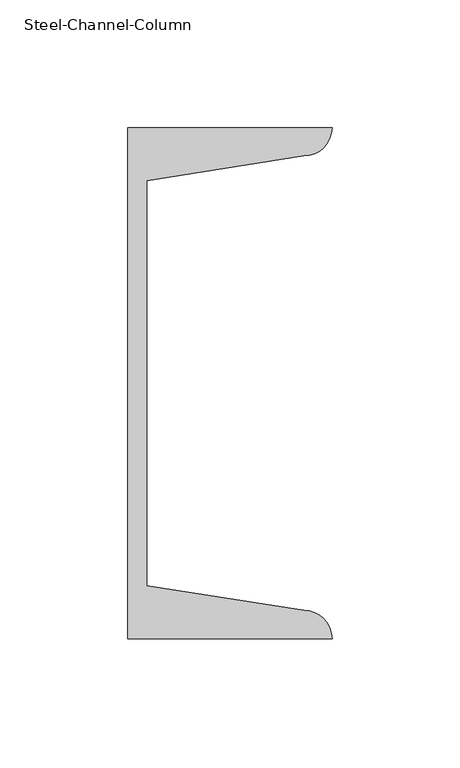
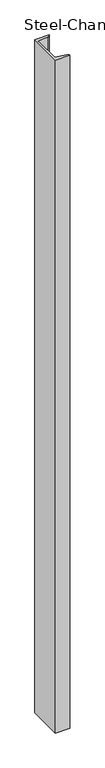
"""IFC4 building model written with IfcOpenShell, lengths in millimetres: column geometry, Steel-Channel-Column : CL126_C-200×80x7.5x11."""

from ifc_helpers import new_model, si_unit, point, frame_2d, origin, origin_with_axes, place, context, project, spatial, polyline, circle_curve, trimmed, segment, composite_curve, outline, extrude, source, transform, mapped, element, save


def steel_channel_column_12e21b6e(model_context):
    return source(origin(), model_context, "Body", "SweptSolid", [
        extrude(outline(composite_curve([segment(polyline([(-22.1, 100.0), (57.9, 100.0)]), True, "CONTINUOUS"), segment(trimmed(circle_curve(frame_2d((46.9, 100.0)), 11.0), [point((57.9, 100.0))], [point((46.9, 89.0))], False, "CARTESIAN"), True, "CONTINUOUS"), segment(polyline([(46.9, 89.0), (-14.6, 79.2593569), (-14.6, -79.2593569), (46.9, -89.0)]), True, "CONTINUOUS"), segment(trimmed(circle_curve(frame_2d((46.9, -100.0)), 11.0), [point((46.9, -89.0))], [point((57.9, -100.0))], False, "CARTESIAN"), True, "CONTINUOUS"), segment(polyline([(57.9, -100.0), (-22.1, -100.0), (-22.1, 100.0)]), True, "CONTINUOUS")], self_intersect=False)), origin_with_axes(), (0.0, 0.0, 1.0), 4000.0),
    ])


if __name__ == "__main__":
    model = new_model("IFC4")
    model_context = context("Model", 3, world=origin())
    ifc_project = project(units=[si_unit("LENGTHUNIT", "METRE", prefix="MILLI")], contexts=[model_context])
    site = spatial("IfcSite", under=ifc_project)
    building = spatial("IfcBuilding", under=site)
    placement = place(None, origin())
    steel_channel_column_shape = steel_channel_column_12e21b6e(model_context)
    element("IfcColumn", 1, ObjectType="Steel-Channel-Column : CL126_C-200×80x7.5x11", at=placement, inside=building, context=model_context, shape_type="MappedRepresentation", body=[
        mapped(steel_channel_column_shape, transform((0.0, 0.0, 0.0), x_axis=(1.0, 0.0, 0.0), y_axis=(0.0, 1.0, 0.0), z_axis=(0.0, 0.0, 1.0))),
    ])
    save(model, "model.ifc")

# Revit data of these elements
# Project information
#   Project ISM Data = "<?xml version=\"1.0\" encoding=\"utf-16\"?><ism schema_version=\"03.00\"><section_positioning><element family_name=\"CO_RC_REC\" symbol_name=\"CCC12_Rec_450x450\" section_id=\"F2ADF140-E21A-4820-8170-6F63D956DCAD\" category=\"OST_StructuralColumns\" mirror_y=\"0\" mirror_x=\"0\" /><element family_name=\"CO_RC_REC\" symbol_name=\"CCC12_Rec_450x450\" section_id=\"B35A310E-4F33-462b-819C-3ADD300C0CEB\" category=\"OST_StructuralColumns\" mirror_y=\"0\" mirror_x=\"0\" /><element family_name=\"CO_RC_REC\" symbol_name=\"CCC12_Rec_450x450\" section_id=\"711054EC-0DB2-46e3-AD20-004560300C00\" category=\"OST_StructuralColumns\" mirror_y=\"0\" mirror_x=\"0\" /><element family_name=\"CO_RC_REC\" symbol_name=\"300 x 450\" section_id=\"B5C54EC9-8EBD-4860-AB72-EF5791AED394\" category=\"OST_StructuralColumns\" mirror_y=\"0\" mirror_x=\"0\" /><element family_name=\"GI_RC_C\" symbol_name=\"SGC11_400x500\" section_id=\"0A7B8D02-9EA4-4aa9-A41A-E30BB5B6B6C5\" category=\"OST_StructuralFraming\" mirror_y=\"0\" mirror_x=\"0\" /><element family_name=\"GI_RC_C\" symbol_name=\"SGC11_400x500\" section_id=\"714BBD27-DB58-47da-B54C-5806291C2D3C\" category=\"OST_StructuralFraming\" mirror_y=\"0\" mirror_x=\"0\" /><element family_name=\"GI_RC_C\" symbol_name=\"SGC11_400x500\" section_id=\"F36E62C1-13EE-4807-A3C1-899E23E0BEDE\" category=\"OST_StructuralFraming\" mirror_y=\"0\" mirror_x=\"0\" /><element family_name=\"GI_RC_C\" symbol_name=\"SGC11_400x500\" section_id=\"F5448801-679E-44d6-8F46-E676344F8165\" category=\"OST_StructuralFraming\" mirror_y=\"0\" mirror_x=\"0\" /><element family_name=\"GI_RC_C\" symbol_name=\"SGC11_400x600\" section_id=\"05D74241-6318-4cac-95F5-7B878260D5B5\" category=\"OST_StructuralFraming\" mirror_y=\"0\" mirror_x=\"0\" /><element family_name=\"GI_RC_C\" symbol_name=\"SGC11_400x500\" section_id=\"846DCB0C-E06B-4978-9D43-E1CC0FDE7595\" category=\"OST_StructuralFraming\" mirror_y=\"0\" mirror_x=\"0\" /><element family_name=\"GI_RC_C\" symbol_name=\"SGC11_400x500\" section_id=\"2ADF82B8-986D-4f44-85DE-89D921292160\" category=\"OST_StructuralFraming\" mirror_y=\"0\" mirror_x=\"0\" /><element family_name=\"GI_RC_C\" symbol_name=\"SGC11_400x500\" section_id=\"7AF371ED-051B-4a30-8826-11F11C212B73\" category=\"OST_StructuralFraming\" mirror_y=\"0\" mirror_x=\"0\" /><element family_name=\"GI_RC_C\" symbol_name=\"SGC11_400x500\" section_id=\"2FE74006-ADDA-412f-A522-853919E62B4D\" category=\"OST_StructuralFraming\" mirror_y=\"0\" mirror_x=\"0\" /><element family_name=\"GI_RC_C\" symbol_name=\"SGC11_400x500\" section_id=\"09B63641-D581-4a6c-A18E-54C17EC989A4\" category=\"OST_StructuralFraming\" mirror_y=\"0\" mirror_x=\"0\" /><element family_name=\"GI_RC_C\" symbol_name=\"SGC11_400x500\" section_id=\"0DD6B52A-77D0-45a1-82B1-8236ED57078C\" category=\"OST_StructuralFraming\" mirror_y=\"0\" mirror_x=\"0\" /><element family_name=\"GI_RC_C\" symbol_name=\"SGC11_400x500\" section_id=\"35D311D2-DEB8-4469-97DE-110B6DF5B84D\" category=\"OST_StructuralFraming\" mirror_y=\"0\" mirror_x=\"0\" /><element family_name=\"GI_RC_C\" symbol_name=\"SGC11_400x500\" section_id=\"0D3CCDE5-CFF9-431b-A4BD-01BF6636D6BD\" category=\"OST_StructuralFraming\" mirror_y=\"0\" mirror_x=\"0\" /><element family_name=\"GI_RC_C\" symbol_name=\"SGC11_400x500\" section_id=\"C62B2A5B-024A-47ac-B030-C17A67E64A7B\" category=\"OST_StructuralFraming\" mirror_y=\"0\" mirror_x=\"0\" /><element family_name=\"GI_RC_C\" symbol_name=\"SGC11_400x500\" section_id=\"944C6E43-E607-48c3-8358-9E6CB88346E7\" category=\"OST_StructuralFraming\" mirror_y=\"0\" mirror_x=\"0\" /><element family_name=\"GI_RC_C\" symbol_name=\"SGC11_400x500\" section_id=\"A4B1F42D-B1C2-4ad2-8AD6-DB0D5E05998D\" category=\"OST_StructuralFraming\" mirror_y=\"0\" mirror_x=\"0\" /><element family_name=\"GI_RC_C\" symbol_name=\"SGC11_400x500\" section_id=\"007E6C70-1139-4b48-B003-C76FAD4C249A\" category=\"OST_StructuralFraming\" mirror_y=\"0\" mirror_x=\"0\" /><element family_name=\"GI_RC_C\" symbol_name=\"SGC11_400x500\" section_id=\"9941AC94-F03A-464c-9912-04590E0C31E0\" category=\"OST_StructuralFraming\" mirror_y=\"0\" mirror_x=\"0\" /><element family_name=\"GI_RC_C\" symbol_name=\"SGC11_400x500\" section_id=\"CFD98B8D-8FF4-4e71-A909-0FE7DBCE924E\" category=\"OST_StructuralFraming\" mirror_y=\"0\" mirror_x=\"0\" /><element family_name=\"GI_RC_C\" symbol_name=\"SGC11_400x500\" section_id=\"58262161-98E6-45c8-B2BD-4508105FF662\" category=\"OST_StructuralFraming\" mirror_y=\"0\" mirror_x=\"0\" /><element family_name=\"GI_RC_C\" symbol_name=\"SGC11_400x500\" section_id=\"66AB4841-610A-4883-97F7-1282A56484E1\" category=\"OST_StructuralFraming\" mirror_y=\"0\" mirror_x=\"0\" /><element family_name=\"GI_RC_C\" symbol_name=\"SGC11_400x500\" section_id=\"D2B324BE-BBD6-49da-9730-60EA7AD4D3A0\" category=\"OST_StructuralFraming\" mirror_y=\"0\" mirror_x=\"0\" /><element family_name=\"GI_RC_C\" symbol_name=\"SGC11_400x500\" section_id=\"92A8ECE7-C053-46b1-92ED-F2C041617E7B\" category=\"OST_StructuralFraming\" mirror_y=\"0\" mirror_x=\"0\" /><element family_name=\"GI_RC_C\" symbol_name=\"SGC11_400x500\" section_id=\"B4C4BDB0-65C4-4016-9C78-DBD77E229523\" category=\"OST_StructuralFraming\" mirror_y=\"0\" mirror_x=\"0\" /><element family_name=\"GI_RC_C\" symbol_name=\"SGC11_400x500\" section_id=\"57270646-162F-4c83-BDB7-A5FBEA9120BD\" category=\"OST_StructuralFraming\" mirror_y=\"0\" mirror_x=\"0\" /><element family_name=\"GI_RC_C\" symbol_name=\"SGC11_400x500\" section_id=\"BDEF733F-00AA-4eee-B6C6-50229FC1D236\" category=\"OST_StructuralFraming\" mirror_y=\"0\" mirror_x=\"0\" /><element family_name=\"GI_RC_C\" symbol_name=\"SGC11_400x500\" section_id=\"84A94E1E-3074-40f4-9690-97191755F019\" category=\"OST_StructuralFraming\" mirror_y=\"0\" mirror_x=\"0\" /><element family_name=\"GI_RC_C\" symbol_name=\"SGC11_400x500\" section_id=\"8A7D913D-7967-4718-912D-B83DF0AD2EDD\" category=\"OST_StructuralFraming\" mirror_y=\"0\" mirror_x=\"0\" /><element family_name=\"GI_RC_C\" symbol_name=\"SGC11_400x500\" section_id=\"83553D70-90FA-469c-B5C3-EF03F3FC6475\" category=\"OST_StructuralFraming\" mirror_y=\"0\" mirror_x=\"0\" /><element family_name=\"GI_RC_C\" symbol_name=\"SGC11_400x500\" section_id=\"6880C1E4-C50B-4c1b-B61C-23F2D8C46873\" category=\"OST_StructuralFraming\" mirror_y=\"0\" mirror_x=\"0\" /><element family_name=\"GI_RC_C\" symbol_name=\"SGC11_400x500\" section_id=\"08594C43-CD40-47de-A3BA-8BFB47F64994\" category=\"OST_StructuralFraming\" mirror_y=\"0\" mirror_x=\"0\" /><element family_name=\"GI_RC_C\" symbol_name=\"SGC11_400x500\" section_id=\"7D2E11FA-A5E1-4434-B9BE-AABA1A16CA03\" category=\"OST_StructuralFraming\" mirror_y=\"0\" mirror_x=\"0\" /><element family_name=\"GI_RC_C\" symbol_name=\"SGC11_400x500\" section_id=\"D892DFA4-5441-4ad2-A390-253492293B1B\" category=\"OST_StructuralFraming\" mirror_y=\"0\" mirror_x=\"0\" /><element family_name=\"GI_RC_C\" symbol_name=\"SGC11_400x500\" section_id=\"E5A32FE6-89C4-49f1-B3B9-1CABE7C48A4D\" category=\"OST_StructuralFraming\" mirror_y=\"0\" mirror_x=\"0\" /><element family_name=\"GI_RC_C\" symbol_name=\"SGC11_400x500\" section_id=\"8AE872C2-5DBE-47c5-934B-7E964A84B589\" category=\"OST_StructuralFraming\" mirror_y=\"0\" mirror_x=\"0\" /><element family_name=\"GI_RC_C\" symbol_name=\"SGC11_400x500\" section_id=\"3C847B60-488A-4604-A400-16A3A65E919B\" category=\"OST_StructuralFraming\" mirror_y=\"0\" mirror_x=\"0\" /><element family_name=\"GI_RC_C\" symbol_name=\"SGC11_400x500\" section_id=\"DBEC432A-3F7B-4266-AD99-2A937DC70BCF\" category=\"OST_StructuralFraming\" mirror_y=\"0\" mirror_x=\"0\" /><element family_name=\"GI_RC_C\" symbol_name=\"SGC11_400x500\" section_id=\"59403DD6-7A51-48aa-A3BE-962457E6F10E\" category=\"OST_StructuralFraming\" mirror_y=\"0\" mirror_x=\"0\" /><element family_name=\"GI_RC_C\" symbol_name=\"SGC11_400x500\" section_id=\"11CDDF5D-38B6-43b2-A291-FC188BE232BC\" category=\"OST_StructuralFraming\" mirror_y=\"0\" mirror_x=\"0\" /><element family_name=\"GI_RC_C\" symbol_name=\"SGC11_400x500\" section_id=\"10BF2843-EFC9-4136-933C-5B270D970277\" category=\"OST_StructuralFraming\" mirror_y=\"0\" mirror_x=\"0\" /><element family_name=\"GI_RC_C\" symbol_name=\"SGC11_400x500\" section_id=\"E1B09A9C-F6C6-47d9-976B-E313C0E3F52B\" category=\"OST_StructuralFraming\" mirror_y=\"0\" mirror_x=\"0\" /><element family_name=\"GI_RC_C\" symbol_name=\"SGC11_400x500\" section_id=\"A3A22EC3-26C8-4588-A0AB-AFAE02DF267E\" category=\"OST_StructuralFraming\" mirror_y=\"0\" mirror_x=\"0\" /><element family_name=\"GI_RC_C\" symbol_name=\"SGC11_400x500\" section_id=\"114828FC-BDC1-4343-9119-BCB5395DAA64\" category=\"OST_StructuralFraming\" mirror_y=\"0\" mirror_x=\"0\" /><element family_name=\"GI_RC_C\" symbol_name=\"SGC11_400x500\" section_id=\"797626F9-3558-4623-826F-15FB93088CB3\" category=\"OST_StructuralFraming\" mirror_y=\"0\" mirror_x=\"0\" /><element family_name=\"GI_RC_C\" symbol_name=\"SGC11_400x500\" section_id=\"4BF369CD-DF09-4346-96CB-C6C6380A2599\" category=\"OST_StructuralFraming\" mirror_y=\"0\" mirror_x=\"0\" /><element family_name=\"GI_RC_C\" symbol_name=\"SGC11_400x500\" section_id=\"722B46BA-61C4-44a1-9ECF-325B60B6688D\" category=\"OST_StructuralFraming\" mirror_y=\"0\" mirror_x=\"0\" /><element family_name=\"GI_RC_C\" symbol_name=\"SGC11_400x500\" section_id=\"C33DBE84-19C1-4379-AB6E-A41F7420F18C\" category=\"OST_StructuralFraming\" mirror_y=\"0\" mirror_x=\"0\" /><element family_name=\"GI_RC_C\" symbol_name=\"SGC11_400x500\" section_id=\"1F2D3B75-66F2-4d88-A1DD-647969477B86\" category=\"OST_StructuralFraming\" mirror_y=\"0\" mirror_x=\"0\" /><element family_name=\"GI_RC_C\" symbol_name=\"SGC11_400x500\" section_id=\"DFBF96B2-410A-4f39-80C4-D8CF78561C93\" category=\"OST_StructuralFraming\" mirror_y=\"0\" mirror_x=\"0\" /><element family_name=\"GI_RC_C\" symbol_name=\"SGC11_400x500\" section_id=\"D6793CD3-AB64-417c-9C28-8B18A0A2D336\" category=\"OST_StructuralFraming\" mirror_y=\"0\" mirror_x=\"0\" /><element family_name=\"GI_RC_C\" symbol_name=\"SGC11_400x500\" section_id=\"90884AC0-EA00-4caa-86E1-E6B886FD90ED\" category=\"OST_StructuralFraming\" mirror_y=\"0\" mirror_x=\"0\" /><element family_name=\"GI_RC_C\" symbol_name=\"SGC11_400x500\" section_id=\"64BC7B89-F7C8-4dae-A5C8-F10DF9E5F6BA\" category=\"OST_StructuralFraming\" mirror_y=\"0\" mirror_x=\"0\" /><element family_name=\"GI_RC_C\" symbol_name=\"SGC11_400x500\" section_id=\"D82E4D85-2728-40e5-9F60-1C7FB2990D78\" category=\"OST_StructuralFraming\" mirror_y=\"0\" mirror_x=\"0\" /><element family_name=\"GI_RC_C\" symbol_name=\"SGC11_400x500\" section_id=\"1E6D05B9-BF84-4669-AA27-948ADA1D511E\" category=\"OST_StructuralFraming\" mirror_y=\"0\" mirror_x=\"0\" /><element family_name=\"GI_RC_C\" symbol_name=\"SGC11_400x500\" section_id=\"73608CB2-EB94-466e-883D-814030EF49D6\" category=\"OST_StructuralFraming\" mirror_y=\"0\" mirror_x=\"0\" /><element family_name=\"GI_RC_C\" symbol_name=\"SGC11_400x500\" section_id=\"4EAF07EF-4E08-4065-9F08-BF69D4413867\" category=\"OST_StructuralFraming\" mirror_y=\"1\" mirror_x=\"1\" /></section_positioning><surface_member_mappings /><element_binding><element revit_id=\"0aa8b22b-49cd-4eb2-b994-d423f7aad482-0014435e\" ism_id=\"637A3C89-B4B9-4EE4-9E04-FF73E7A5771D\" /><element revit_id=\"af7cfdda-f71a-4a09-bb03-63e0c16d5d93-00152efa\" ism_id=\"088C1743-AFAE-4D55-B14F-2330F3A79060\" /><element revit_id=\"af7cfdda-f71a-4a09-bb03-63e0c16d5d93-00152efc\" ism_id=\"38278b30-864a-4bde-bfee-6c2d4309b281\" /><element revit_id=\"af7cfdda-f71a-4a09-bb03-63e0c16d5d93-00152eff\" ism_id=\"e2895b00-887b-4cf1-92a9-c4855f67b579\" /><element revit_id=\"af7cfdda-f71a-4a09-bb03-63e0c16d5d93-00152f02\" ism_id=\"a6b13b86-1938-47ee-8937-754844bb71d9\" /><element revit_id=\"af7cfdda-f71a-4a09-bb03-63e0c16d5d93-00152f05\" ism_id=\"b3cdb4ae-01be-49a8-8521-dfb37fcb7a09\" /><element revit_id=\"af7cfdda-f71a-4a09-bb03-63e0c16d5d93-00152f08\" ism_id=\"0a200294-2d0f-43b2-a10b-c345be42008c\" /><element revit_id=\"af7cfdda-f71a-4a09-bb03-63e0c16d5d
#     93-00152f0a\" ism_id=\"434ac00d-0b75-408a-b526-bf8655b26baf\" /><element revit_id=\"af7cfdda-f71a-4a09-bb03-63e0c16d5d93-00152f0c\" ism_id=\"5e4f7e2a-2154-47cc-93bc-24e7bd197632\" /><element revit_id=\"af7cfdda-f71a-4a09-bb03-63e0c16d5d93-00152f0e\" ism_id=\"f1998cd9-044c-4f7a-99e6-248bc5b45dba\" /><element revit_id=\"af7cfdda-f71a-4a09-bb03-63e0c16d5d93-00152f10\" ism_id=\"6ca0e144-6dd7-4824-b6a4-c3599ffcc64c\" /><element revit_id=\"af7cfdda-f71a-4a09-bb03-63e0c16d5d93-00152f12\" ism_id=\"173f1f07-ca52-4750-b7f6-1ef0180c36ba\" /><element revit_id=\"af7cfdda-f71a-4a09-bb03-63e0c16d5d93-00152f15\" ism_id=\"29a619d1-86ac-46c7-a220-2e78769b313e\" /><element revit_id=\"af7cfdda-f71a-4a09-bb03-63e0c16d5d93-00152f17\" ism_id=\"de21b25d-6b5e-4da6-89ee-8b671f1287ec\" /><element revit_id=\"af7cfdda-f71a-4a09-bb03-63e0c16d5d93-00152f19\" ism_id=\"70cdf538-eeaa-48c4-9315-181e56578638\" /><element revit_id=\"af7cfdda-f71a-4a09-bb03-63e0c16d5d93-00152f1b\" ism_id=\"49734cf8-a963-4163-b104-a25bff74fff0\" /><element revit_id=\"af7cfdda-f71a-4a09-bb03-63e0c16d5d93-00152f1d\" ism_id=\"a5a98e28-e98d-4759-bcab-d40632bfc19f\" /><element revit_id=\"af7cfdda-f71a-4a09-bb03-63e0c16d5d93-00152f1f\" ism_id=\"ab6af08f-90da-4d2f-a66a-db65621b8e94\" /><element revit_id=\"af7cfdda-f71a-4a09-bb03-63e0c16d5d93-00152f21\" ism_id=\"a65b64ab-134d-4223-82b7-5e66d90bc276\" /><element revit_id=\"af7cfdda-f71a-4a09-bb03-63e0c16d5d93-00152f23\" ism_id=\"6a1f317f-8940-4af8-9522-8e6c47c0c3a6\" /><element revit_id=\"af7cfdda-f71a-4a09-bb03-63e0c16d5d93-00152f25\" ism_id=\"880c6aab-7058-4382-9d83-6c759bdcf822\" /><element revit_id=\"af7cfdda-f71a-4a09-bb03-63e0c16d5d93-00152f27\" ism_id=\"555977b1-6494-4ee8-b235-8bae97762787\" /><element revit_id=\"af7cfdda-f71a-4a09-bb03-63e0c16d5d93-00152f29\" ism_id=\"66c9b467-8c65-4f1e-9542-95b43d793e9b\" /><element revit_id=\"af7cfdda-f71a-4a09-bb03-63e0c16d5d93-00152f2b\" ism_id=\"217a9ce2-64ab-4115-836e-06014fa1b21e\" /><element revit_id=\"af7cfdda-f71a-4a09-bb03-63e0c16d5d93-00152f2d\" ism_id=\"f7fc30da-832d-44e7-bab3-dd115d25639e\" /><element revit_id=\"af7cfdda-f71a-4a09-bb03-63e0c16d5d93-00152f2f\" ism_id=\"715eb46c-1b8d-4226-a7c6-6c6c165bf34d\" /><element revit_id=\"af7cfdda-f71a-4a09-bb03-63e0c16d5d93-00152f31\" ism_id=\"ef53c2b2-6fcf-42d2-96ea-f30a899bf64f\" /><element revit_id=\"af7cfdda-f71a-4a09-bb03-63e0c16d5d93-00152f34\" ism_id=\"1aefa093-18ee-4a97-8178-1b1fb4b7aceb\" /><element revit_id=\"af7cfdda-f71a-4a09-bb03-63e0c16d5d93-00152f38\" ism_id=\"262f02a9-64ca-487b-befd-4b58d44dffa7\" /><element revit_id=\"af7cfdda-f71a-4a09-bb03-63e0c16d5d93-00152f3b\" ism_id=\"6f2442a8-c4c0-4b53-9d7f-7059d6ededd2\" /><element revit_id=\"af7cfdda-f71a-4a09-bb03-63e0c16d5d93-00152f3e\" ism_id=\"dd838df4-69c7-406c-93e1-418c01f5734f\" /><element revit_id=\"af7cfdda-f71a-4a09-bb03-63e0c16d5d93-00152f40\" ism_id=\"9dec5077-28a7-4c32-95d2-08813de6a916\" /><element revit_id=\"af7cfdda-f71a-4a09-bb03-63e0c16d5d93-00152f42\" ism_id=\"9370ae5f-9277-4bb3-917b-cb3f318800a8\" /><element revit_id=\"af7cfdda-f71a-4a09-bb03-63e0c16d5d93-00152f44\" ism_id=\"0f3f2c81-58b4-4698-b1be-75061a4a2ae1\" /><element revit_id=\"af7cfdda-f71a-4a09-bb03-63e0c16d5d93-00152f46\" ism_id=\"95dca10f-6510-4ae7-a23e-7a1fd6939662\" /><element revit_id=\"af7cfdda-f71a-4a09-bb03-63e0c16d5d93-00152f49\" ism_id=\"83bad907-6a1c-4702-9990-a1a9c13d0160\" /><element revit_id=\"af7cfdda-f71a-4a09-bb03-63e0c16d5d93-00152f4d\" ism_id=\"7dba72dc-0de8-457c-8d3c-9c80941133ff\" /><element revit_id=\"af7cfdda-f71a-4a09-bb03-63e0c16d5d93-00152f51\" ism_id=\"a6cf3de2-949b-45b4-8029-061e06e5ab91\" /><element revit_id=\"af7cfdda-f71a-4a09-bb03-63e0c16d5d93-00152f54\" ism_id=\"77af5754-dd62-4c90-accb-d0b9405b5baf\" /><element revit_id=\"af7cfdda-f71a-4a09-bb03-63e0c16d5d93-00152f56\" ism_id=\"6461cb37-823d-49bb-bea2-3dbd4db85a81\" /><element revit_id=\"af7cfdda-f71a-4a09-bb03-63e0c16d5d93-00152f59\" ism_id=\"e2f2909f-27bc-426e-b2db-27b1217d3560\" /><element revit_id=\"af7cfdda-f71a-4a09-bb03-63e0c16d5d93-00152f5b\" ism_id=\"46c410de-fc65-4593-ae24-da1a154b45fb\" /><element revit_id=\"af7cfdda-f71a-4a09-bb03-63e0c16d5d93-00152f5d\" ism_id=\"d7d73cf7-a31f-421c-bc39-3ba338a334b1\" /><element revit_id=\"af7cfdda-f71a-4a09-bb03-63e0c16d5d93-00152f61\" ism_id=\"6bd81f7b-5fd8-4f19-ad3a-4e009274854c\" /><element revit_id=\"af7cfdda-f71a-4a09-bb03-63e0c16d5d93-00152f64\" ism_id=\"f25b9af0-504f-4aaf-a359-d2bc9d32b683\" /><element revit_id=\"af7cfdda-f71a-4a09-bb03-63e0c16d5d93-00152f66\" ism_id=\"f143dcd3-1cc7-47ae-b4ed-c960a7d1349c\" /><element revit_id=\"af7cfdda-f71a-4a09-bb03-63e0c16d5d93-00152f68\" ism_id=\"296e8d7f-a89b-405a-b793-fc1ea4b11be5\" /><element revit_id=\"af7cfdda-f71a-4a09-bb03-63e0c16d5d93-00152f6b\" ism_id=\"48b24488-3184-439c-b285-73e81edfef17\" /><element revit_id=\"af7cfdda-f71a-4a09-bb03-63e0c16d5d93-00152f6e\" ism_id=\"0db0ccd4-631c-4972-aad8-2fd483c55629\" /><element revit_id=\"af7cfdda-f71a-4a09-bb03-63e0c16d5d93-00152f71\" ism_id=\"ee51bd40-01d8-4a48-92c6-90509a96cad2\" /><element revit_id=\"af7cfdda-f71a-4a09-bb03-63e0c16d5d93-00152f73\" ism_id=\"e5c66ce6-ca9d-4591-9d75-5348307a88bc\" /><element revit_id=\"af7cfdda-f71a-4a09-bb03-63e0c16d5d93-00152f75\" ism_id=\"892d82ae-6f73-4af5-8575-78955f2b6c3b\" /><element revit_id=\"af7cfdda-f71a-4a09-bb03-63e0c16d5d93-00152f78\" ism_id=\"cb5b2a2e-5551-4b87-9d0b-6382c09e6ce2\" /><element revit_id=\"af7cfdda-f71a-4a09-bb03-63e0c16d5d93-00152f7c\" ism_id=\"1177c4ab-d04b-426b-80ba-afa1f1403e20\" /><element revit_id=\"af7cfdda-f71a-4a09-bb03-63e0c16d5d93-00152f7f\" ism_id=\"235d8a18-f10a-44ad-8945-ebb2f02646fa\" /><element revit_id=\"af7cfdda-f71a-4a09-bb03-63e0c16d5d93-00152f83\" ism_id=\"6127db9d-7d4b-44c8-806c-e4f7d278db0c\" /><element revit_id=\"af7cfdda-f71a-4a09-bb03-63e0c16d5d93-00152f86\" ism_id=\"85d79da8-d317-4e5b-88a2-88d20cb73d7d\" /><element revit_id=\"af7cfdda-f71a-4a09-bb03-63e0c16d5d93-00152f89\" ism_id=\"f4105a19-7c5e-4970-9446-50e578b67af2\" /><element revit_id=\"af7cfdda-f71a-4a09-bb03-63e0c16d5d93-00152f8b\" ism_id=\"ab299061-87b1-4edc-8a5c-c55542368f39\" /><element revit_id=\"af7cfdda-f71a-4a09-bb03-63e0c16d5d93-00152f8d\" ism_id=\"43097401-25be-48d4-a7ba-f3c37c1b84e9\" /><element revit_id=\"af7cfdda-f71a-4a09-bb03-63e0c16d5d93-00152f8f\" ism_id=\"fd9214b7-59e9-4736-b544-a37d4c180e24\" /><element revit_id=\"af7cfdda-f71a-4a09-bb03-63e0c16d5d93-00152f91\" ism_id=\"b83d1d95-2d97-4532-8a94-368577601c17\" /><element revit_id=\"af7cfdda-f71a-4a09-bb03-63e0c16d5d93-00152f94\" ism_id=\"9bd5e620-e2eb-4ede-9a8b-b0183e171248\" /><element revit_id=\"af7cfdda-f71a-4a09-bb03-63e0c16d5d93-00152f97\" ism_id=\"d6f9d903-1605-43dc-872c-2f9de6642af6\" /><element revit_id=\"af7cfdda-f71a-4a09-bb03-63e0c16d5d93-00152f99\" ism_id=\"7c236b12-3da8-4ae0-bc99-2aa089118476\" /><element revit_id=\"af7cfdda-f71a-4a09-bb03-63e0c16d5d93-00152f9b\" ism_id=\"2b88d03d-aeef-4f51-b98c-562513d6f6da\" /><element revit_id=\"af7cfdda-f71a-4a09-bb03-63e0c16d5d93-00152f9d\" ism_id=\"6639b07f-6759-4580-bc0a-91cdbc82216d\" /><element revit_id=\"af7cfdda-f71a-4a09-bb03-63e0c16d5d93-00152f9f\" ism_id=\"d17e7cf5-d760-4c38-8bb0-8a57fe45e3ad\" /><element revit_id=\"af7cfdda-f71a-4a09-bb03-63e0c16d5d93-00152fa2\" ism_id=\"6dbdf2a2-22ac-4132-a9ae-8992fe15b0d7\" /><element revit_id=\"af7cfdda-f71a-4a09-bb03-63e0c16d5d93-00152fa4\" ism_id=\"663381be-9f3f-499f-b7c1-64170401ecb3\" /><element revit_id=\"af7cfdda-f71a-4a09-bb03-63e0c16d5d93-00152fa6\" ism_id=\"5ba3ff14-3d24-47a8-9418-aecce16bd943\" /><element revit_id=\"af7cfdda-f71a-4a09-bb03-63e0c16d5d93-00152fa8\" ism_id=\"8f845e6a-1432-4c61-8362-e12c105320fb\" /><element revit_id=\"af7cfdda-f71a-4a09-bb03-63e0c16d5d93-00152faa\" ism_id=\"263897bf-02c2-4ed7-8e3f-2020d545125e\" /><element revit_id=\"af7cfdda-f71a-4a09-bb03-63e0c16d5d93-00152fac\" ism_id=\"f1241312-d990-4c87-92ff-afc1975a3d67\" /><element revit_id=\"af7cfdda-f71a-4a09-bb03-63e0c16d5d93-00152fae\" ism_id=\"5740cb23-0cbc-47ce-acea-31b5a043bf0c\" /><element revit_id=\"af7cfdda-f71a-4a09-bb03-63e0c16d5d93-00152fb0\" ism_id=\"7aeaeafb-f9bc-4bee-b237-caade22069b8\" /><element revit_id=\"af7cfdda-f71a-4a09-bb03-63e0c16d5d93-00152fb3\" ism_id=\"90084dda-e197-4e46-8e5b-4f629a594830\" /><element revit_id=\"af7cfdda-f71a-4a09-bb03-63e0c16d5d93-00152fb5\" ism_id=\"2c392f12-2b50-4bd2-8c41-ef64640e587b\" /><element revit_id=\"af7cfdda-f71a-4a09-bb03-63e0c16d5d93-00152fb7\" ism_id=\"d25284c0-6931-4cbb-8ed3-63397f6a5616\" /><element revit_id=\"af7cfdda-f71a-4a09-bb03-63e0c16d5d93-00152fb9\" ism_id=\"32799d39-e9bc-468c-ac64-a3f2c8e075af\" /><element revit_id=\"af7cfdda-f71a-4a09-bb03-63e0c16d5d93-00152fbb\" ism_id=\"61a092b8-d924-4e61-a1ef-adc051541aaf\" /><element revit_id=\"af7cfdda-f71a-4a09-bb03-63e0c16d5d93-00152fbe\" ism_id=\"ae89ad42-0006-42ee-9328-01a896002b7a\" /><element revit_id=\"af7cfdda-f71a-4a09-bb03-63e0c16d5d93-00152fc0\" ism_id=\"7b4d47fd-5fcd-4692-9b39-36bb95372647\" /><element revit_id=\"af7cfdda-f71a-4a09-bb03-63e0c16d5d93-00152fc2\" ism_id=\"150f022d-eb78-47d8-8d70-c7ea5433f366\" /><element revit_id=\"af7cfdda-f71a-4a09-bb03-63e0c16d5d93-00152fc4\" ism_id=\"6780451e-52c6-4962-8bb4-f1fd57bf7865\" /><element revit_id=\"af7cfdda-f71a-4a09-bb03-63e0c16d5d93-00152fc6\" ism_id=\"b3896748-2d7c-424b-ae81-8b769d840fbc\" /><element revit_id=\"af7cfdda-f71a-4a09-bb03-63e0c16d5d93-00152fc9\" ism_id=\"0c64c745-ce95-4f37-8a9d-d07fd5d17ecb\" /><element revit_id=\"af7cfdda-f71a-4a09-bb03-63e0c16d5d93-00152fcc\" ism_id=\"dc23390d-d501-4d7e-9369-f7793a7306a7\" /><element revit_id=\"af7cfdda-f71a-4a09-bb03-63e0c16d5d93-00152fcf\" ism_id=\"a2d2dfc7-08e7-459b-9de9-2d46c1b9d65d\" /><element revit_id=\"af7cfdda-f71a-4a09-bb03-63e0c16d5d93-00152fd2\" ism_id=\"0357c393-c221-46b8-a525-7eece05024d5\" /><element revit_id=\"af7cfdda-f71a-4a09-bb03-63e0c16d5d93-00152fd4\" ism_id=\"7514ec1a-cc54-428f-bbfe-53465c7b9971\" /><element revit_id=\"af7cfdda-f71a-4a09-bb03-63e0c16d5d93-00152fd7\" ism_id=\"f5e61f1a-565d-4eed-b8cc-74798bf49f83\" /><element revit_id=\"af7cfdda-f71a-4a09-bb03-63e0c16d5d93-00152fd9\" ism_id=\"7d7031a0-6061-49e6-8bb3-df1503ddb602\" /><element revit_id=\"af7cfdda-f71a-4a09-bb03-63e0c16d5d93-00152fdb\" ism_id=\"0d733cbc-e2dd-44ec-a5f3-da43d2d7ec46\" /><element revit_id=\"af7cfdda-f71a-4a09-bb03-63e0c16d5d93-00152fdd\" ism_id=\"21cbc8e9-c640-4a2e-8958-1d3b7a784879\" /><element revit_id=\"af7cfdda-f71a-4a09-bb03-63e0c16d5d93-00152fdf\" ism_id=\"fac86bbb-1d81-4320-81cd-30997be31eb4\" /><element revit_id=\"af7cfdda-f71a-4a09-bb03-63e0c16d5d93-00152fe1\" ism_id=\"ebc7c696-170e-4ba4-8599-103279d331b8\" /><element revit_id=\"af7cfdda-f71a-4a09-bb03-63e0c16d5d93-00152fe3\" ism_id=\"91dec439-7fd8-4259-bbce-df46237765e2\" /><element revit_id=\"af7cfdda-f71a-4a09-bb03-63e0c16d5d93-00152fe5\" ism_id=\"6227503a-c521-4b5a-b5c3-b9e2ea2b5c81\" /><element revit_id=\"af7cfdda-f71a-4a09-bb03-63e0c16d5d93-00152fe7\" ism_id=\"e6e91966-53ab-4536-84a0-3f6e5a22fbeb\" /><element revit_id=\"af7cfdda-f71a-4a09-bb03-63e0c16d5d93-00152fe9\" ism_id=\"fb3387b3-301c-40a5-8217-97be67c50843\" /><element revit_id=\"af7cfdda-f71a-4a09-bb03-63e0c16d5d93-00152feb\" ism_id=\"37825fc8-0fe2-440e-933a-1453c922c9d9\" /><element revit_id=\"af7cfdda-f71a-4a09-bb03-63e0c16d5d93-00152fed\" ism_id=\"06b175df-5526-4920-a3d6-7f2ff872756e\" /><element revit_id=\"af7cfdda-f71a-4a09-bb03-63e0c16d5d93-00152fef\" ism_id=\"a8fbce7a-6989-46e5-9bc5-c497d4a295c9\" /><element revit_id=\"af7cfdda-f71a-4a09-bb03-63e0c16d5d93-00152ff1\" ism_id=\"cf8ccf89-d0da-4b4e-93d8-85d639853d5e\" /><element revit_id=\"af7cfdda-f71a-4a09-bb03-63e0c16d5d93-00152ff3\" ism_id=\"1b85e87c-6c2a-4057-8491-40e4237cd0e6\" /><element revit_id=\"af7cfdda-f71a-4a09-bb03-63e0c16d5d93-00152ff5\" ism_id=\"69be497f-343c-4d38-9ea0-e959474332f8\" /><element revit_id=\"af7cfdda-f71a-4a09-bb03-63e0c16d5d93-00152ff7\" ism_id=\"72738956-f87a-41b4-a019-35adc3bff764\" /><element revit_id=\"af7cfdda-f71a-4a09-bb03-63e0c16d5d93-00152ff9\" ism_id=\"f127b15c-142d-4b57-83a6-5b76ac4cde6e\" /><element revit_id=
#     \"af7cfdda-f71a-4a09-bb03-63e0c16d5d93-00152ffb\" ism_id=\"3a38a709-bfa8-404e-b889-5af5e78ea0bf\" /><element revit_id=\"af7cfdda-f71a-4a09-bb03-63e0c16d5d93-00152ffe\" ism_id=\"bebf0363-7e59-4a43-8f5b-502fcc4a338d\" /><element revit_id=\"af7cfdda-f71a-4a09-bb03-63e0c16d5d93-00153000\" ism_id=\"157fe154-0d28-4e8c-a143-e2896867fd28\" /><element revit_id=\"af7cfdda-f71a-4a09-bb03-63e0c16d5d93-00153002\" ism_id=\"1bf52bf8-7327-4d55-b5cd-bf7c9bf89688\" /><element revit_id=\"af7cfdda-f71a-4a09-bb03-63e0c16d5d93-00153005\" ism_id=\"7a0025bf-d54b-4614-9002-7bd4a82da90e\" /><element revit_id=\"af7cfdda-f71a-4a09-bb03-63e0c16d5d93-00153008\" ism_id=\"cad53638-8c8f-4a89-ab6f-d8a32131833b\" /><element revit_id=\"af7cfdda-f71a-4a09-bb03-63e0c16d5d93-0015300a\" ism_id=\"05672ccd-1a96-434c-8da1-7a706b3561f7\" /><element revit_id=\"af7cfdda-f71a-4a09-bb03-63e0c16d5d93-0015300c\" ism_id=\"bb809016-b2bb-4157-847e-1cca3692ba19\" /><element revit_id=\"af7cfdda-f71a-4a09-bb03-63e0c16d5d93-0015300f\" ism_id=\"720ed192-8aa7-46fd-9f7a-15d64351767c\" /><element revit_id=\"af7cfdda-f71a-4a09-bb03-63e0c16d5d93-00153011\" ism_id=\"9a47cdb9-976d-41f3-a5c3-5a7516a7763c\" /><element revit_id=\"af7cfdda-f71a-4a09-bb03-63e0c16d5d93-00153013\" ism_id=\"aba01787-c82b-453e-8db2-70277a34d5ad\" /><element revit_id=\"af7cfdda-f71a-4a09-bb03-63e0c16d5d93-00153015\" ism_id=\"f6b882e3-d64a-44b1-878c-9c00ee1fde86\" /><element revit_id=\"af7cfdda-f71a-4a09-bb03-63e0c16d5d93-00153017\" ism_id=\"95108815-490a-427a-aec1-8fcefc57c858\" /><element revit_id=\"af7cfdda-f71a-4a09-bb03-63e0c16d5d93-00153019\" ism_id=\"8fe55cf1-56b4-4a62-948a-d7f0c95bd04b\" /><element revit_id=\"af7cfdda-f71a-4a09-bb03-63e0c16d5d93-0015301b\" ism_id=\"b889bf8b-3bdd-410a-b11b-9ca69449d470\" /><element revit_id=\"af7cfdda-f71a-4a09-bb03-63e0c16d5d93-0015301d\" ism_id=\"ef8604de-de5b-45ec-9158-0b702e6ef713\" /><element revit_id=\"af7cfdda-f71a-4a09-bb03-63e0c16d5d93-0015301f\" ism_id=\"40ee286a-4bc9-4d4f-ba6d-fe1ac9da03cf\" /><element revit_id=\"af7cfdda-f71a-4a09-bb03-63e0c16d5d93-00153021\" ism_id=\"cc903f39-6bdf-4081-a56c-883169221735\" /><element revit_id=\"af7cfdda-f71a-4a09-bb03-63e0c16d5d93-00153023\" ism_id=\"0af04955-dcb6-4295-b3d4-7c432a233062\" /><element revit_id=\"af7cfdda-f71a-4a09-bb03-63e0c16d5d93-00153025\" ism_id=\"75a51549-6a04-4399-b818-f170a8c10286\" /><element revit_id=\"af7cfdda-f71a-4a09-bb03-63e0c16d5d93-00153027\" ism_id=\"7e183794-5c66-46bc-97f5-2df209b3286d\" /><element revit_id=\"af7cfdda-f71a-4a09-bb03-63e0c16d5d93-00153029\" ism_id=\"ed4a7448-29b0-44e3-8b6f-7310f83440ab\" /><element revit_id=\"af7cfdda-f71a-4a09-bb03-63e0c16d5d93-0015302b\" ism_id=\"fdb5eb17-b94e-40c1-b703-3ecb5e4efee4\" /><element revit_id=\"af7cfdda-f71a-4a09-bb03-63e0c16d5d93-0015302d\" ism_id=\"779397c1-65b7-447f-a72e-2a09308021ea\" /><element revit_id=\"af7cfdda-f71a-4a09-bb03-63e0c16d5d93-0015302f\" ism_id=\"7b409707-86c5-44e2-919e-92ad5bb9eb8b\" /><element revit_id=\"af7cfdda-f71a-4a09-bb03-63e0c16d5d93-00153031\" ism_id=\"d337c78b-590d-406c-bf20-6a3558821db1\" /><element revit_id=\"af7cfdda-f71a-4a09-bb03-63e0c16d5d93-00153033\" ism_id=\"c27f5f6d-8445-4415-853d-d316787bea6e\" /><element revit_id=\"af7cfdda-f71a-4a09-bb03-63e0c16d5d93-00153035\" ism_id=\"76036a55-3bab-417a-ba41-ec1335e2e2a7\" /><element revit_id=\"af7cfdda-f71a-4a09-bb03-63e0c16d5d93-00153037\" ism_id=\"24be638c-ff89-4616-8974-5b79c81e6e56\" /><element revit_id=\"af7cfdda-f71a-4a09-bb03-63e0c16d5d93-00153039\" ism_id=\"015f9f2c-2353-4795-b891-e4ee986f25f7\" /><element revit_id=\"af7cfdda-f71a-4a09-bb03-63e0c16d5d93-0015303b\" ism_id=\"91f8ddfb-c5b9-4f33-b141-a6edfbccf098\" /><element revit_id=\"af7cfdda-f71a-4a09-bb03-63e0c16d5d93-0015303d\" ism_id=\"78540364-1ba5-4f0c-95fb-ba8631e32695\" /><element revit_id=\"af7cfdda-f71a-4a09-bb03-63e0c16d5d93-0015303f\" ism_id=\"9d53e406-367b-4e3e-b5e8-d421731e1aab\" /><element revit_id=\"af7cfdda-f71a-4a09-bb03-63e0c16d5d93-00153041\" ism_id=\"24aa6051-1a20-4f08-8962-6f6f9ff4dc98\" /><element revit_id=\"af7cfdda-f71a-4a09-bb03-63e0c16d5d93-00153043\" ism_id=\"572a4144-5250-4962-a1b9-09502cda2774\" /><element revit_id=\"af7cfdda-f71a-4a09-bb03-63e0c16d5d93-00153045\" ism_id=\"1f486980-0be9-4aad-b32e-0608218bf68e\" /><element revit_id=\"af7cfdda-f71a-4a09-bb03-63e0c16d5d93-00153047\" ism_id=\"588ed856-d113-4521-b97c-a4d7ac7ba406\" /><element revit_id=\"af7cfdda-f71a-4a09-bb03-63e0c16d5d93-00153049\" ism_id=\"741942b7-995d-48cb-8401-4faec8ef8d15\" /><element revit_id=\"af7cfdda-f71a-4a09-bb03-63e0c16d5d93-0015304b\" ism_id=\"85254c30-08c9-46e3-acd6-6b5131f485ce\" /><element revit_id=\"af7cfdda-f71a-4a09-bb03-63e0c16d5d93-0015304e\" ism_id=\"2d57d6c0-67d8-48bd-b16f-8ef7edb485b1\" /><element revit_id=\"af7cfdda-f71a-4a09-bb03-63e0c16d5d93-00153050\" ism_id=\"57b4caff-473e-4ebc-b42c-d73ce4ca67d8\" /><element revit_id=\"af7cfdda-f71a-4a09-bb03-63e0c16d5d93-00153052\" ism_id=\"1adae240-a487-478c-a898-61bee40e7415\" /><element revit_id=\"af7cfdda-f71a-4a09-bb03-63e0c16d5d93-00153054\" ism_id=\"62613b5f-092e-4f63-86ac-d3e070a85bc5\" /><element revit_id=\"af7cfdda-f71a-4a09-bb03-63e0c16d5d93-00153056\" ism_id=\"6aecb1de-b991-4eed-80ad-e1b9ccc03a87\" /><element revit_id=\"af7cfdda-f71a-4a09-bb03-63e0c16d5d93-00153058\" ism_id=\"ecab5d8d-84d0-44a4-9549-bca959ac514b\" /><element revit_id=\"af7cfdda-f71a-4a09-bb03-63e0c16d5d93-0015305a\" ism_id=\"589f44ad-061b-46bc-91bd-bf9b1e708415\" /><element revit_id=\"af7cfdda-f71a-4a09-bb03-63e0c16d5d93-0015305c\" ism_id=\"bfa24af8-499f-45ff-9e9d-d5cc0761fed6\" /><element revit_id=\"af7cfdda-f71a-4a09-bb03-63e0c16d5d93-0015305e\" ism_id=\"8114f473-ca73-4cc8-b3e2-979f07368f66\" /><element revit_id=\"af7cfdda-f71a-4a09-bb03-63e0c16d5d93-00153060\" ism_id=\"4dde7439-2ac9-412f-a5f5-e9fd0f294ec8\" /><element revit_id=\"af7cfdda-f71a-4a09-bb03-63e0c16d5d93-00153062\" ism_id=\"661cc7d8-fd9c-4505-b43e-241bfd24b2d0\" /><element revit_id=\"af7cfdda-f71a-4a09-bb03-63e0c16d5d93-00153064\" ism_id=\"1e7f186f-1b55-4d4c-bf9f-18595049605e\" /><element revit_id=\"af7cfdda-f71a-4a09-bb03-63e0c16d5d93-00153066\" ism_id=\"ee968183-c9c6-4eab-86cf-0eda12de724b\" /><element revit_id=\"af7cfdda-f71a-4a09-bb03-63e0c16d5d93-00153068\" ism_id=\"5de1f319-cdd1-4b9a-8f8e-b86394effa22\" /><element revit_id=\"af7cfdda-f71a-4a09-bb03-63e0c16d5d93-0015306a\" ism_id=\"fa557a6c-2e39-4481-9eb5-5ede8fd31c49\" /><element revit_id=\"af7cfdda-f71a-4a09-bb03-63e0c16d5d93-0015306c\" ism_id=\"b2710e8e-0f5f-4e74-a366-aef04da22cd3\" /><element revit_id=\"af7cfdda-f71a-4a09-bb03-63e0c16d5d93-0015306e\" ism_id=\"5633c3b7-f903-46ee-b126-8a20a9a62c90\" /><element revit_id=\"af7cfdda-f71a-4a09-bb03-63e0c16d5d93-00153070\" ism_id=\"62796ef8-c4bb-4b9f-bd14-cc7392046eb4\" /><element revit_id=\"af7cfdda-f71a-4a09-bb03-63e0c16d5d93-00153072\" ism_id=\"db898ada-150e-4ff5-a9f8-16e27b46b754\" /><element revit_id=\"af7cfdda-f71a-4a09-bb03-63e0c16d5d93-00153075\" ism_id=\"d3965d2d-e119-4f6b-af8d-52c8a5397d36\" /><element revit_id=\"af7cfdda-f71a-4a09-bb03-63e0c16d5d93-00153077\" ism_id=\"063574e4-6319-4ba7-8e34-1638a1357d5f\" /><element revit_id=\"af7cfdda-f71a-4a09-bb03-63e0c16d5d93-00153079\" ism_id=\"6de69805-8980-44f0-9316-6d50d1b47cbb\" /><element revit_id=\"af7cfdda-f71a-4a09-bb03-63e0c16d5d93-0015307b\" ism_id=\"e5f77c5b-4806-4993-8875-6149db708e42\" /><element revit_id=\"af7cfdda-f71a-4a09-bb03-63e0c16d5d93-0015307d\" ism_id=\"a13071c9-c086-4896-95a6-a015bc531f25\" /><element revit_id=\"af7cfdda-f71a-4a09-bb03-63e0c16d5d93-0015307f\" ism_id=\"c9d216f9-adca-4752-b8c1-d779727505dd\" /><element revit_id=\"af7cfdda-f71a-4a09-bb03-63e0c16d5d93-00153081\" ism_id=\"5b167621-3850-4169-8bee-1e0420bf6050\" /><element revit_id=\"af7cfdda-f71a-4a09-bb03-63e0c16d5d93-00153083\" ism_id=\"09cf76ae-a083-4203-a622-7e9424374f66\" /><element revit_id=\"af7cfdda-f71a-4a09-bb03-63e0c16d5d93-00153085\" ism_id=\"14063b50-058d-464a-aa08-369865983eeb\" /><element revit_id=\"af7cfdda-f71a-4a09-bb03-63e0c16d5d93-00153087\" ism_id=\"add5837f-63be-4349-b708-9f4051059e25\" /><element revit_id=\"af7cfdda-f71a-4a09-bb03-63e0c16d5d93-00153089\" ism_id=\"b4c60bd3-61cb-423f-916a-fa2b71585228\" /><element revit_id=\"af7cfdda-f71a-4a09-bb03-63e0c16d5d93-0015308b\" ism_id=\"6251d90e-381f-4771-818c-f7465ae91864\" /><element revit_id=\"af7cfdda-f71a-4a09-bb03-63e0c16d5d93-0015308d\" ism_id=\"7693be9d-48ca-4005-bed4-90e9c08d3a38\" /><element revit_id=\"af7cfdda-f71a-4a09-bb03-63e0c16d5d93-0015308f\" ism_id=\"a6a39ca9-cd56-43ba-bfe8-2cf3b78878cc\" /><element revit_id=\"af7cfdda-f71a-4a09-bb03-63e0c16d5d93-00153091\" ism_id=\"1a3956c4-77bb-4ccc-a12d-c3514cf365d4\" /><element revit_id=\"af7cfdda-f71a-4a09-bb03-63e0c16d5d93-00153093\" ism_id=\"2ffa7a89-8ee9-470a-b3d8-7c27f566e226\" /><element revit_id=\"af7cfdda-f71a-4a09-bb03-63e0c16d5d93-00153095\" ism_id=\"e865b460-944f-4057-a6e8-4e39cb88d97d\" /><element revit_id=\"af7cfdda-f71a-4a09-bb03-63e0c16d5d93-00153097\" ism_id=\"69410bb9-8440-4a88-9151-b5459095fe2e\" /><element revit_id=\"af7cfdda-f71a-4a09-bb03-63e0c16d5d93-00153099\" ism_id=\"1efae87b-0246-432c-a428-82c87fb3929c\" /><element revit_id=\"af7cfdda-f71a-4a09-bb03-63e0c16d5d93-0015309b\" ism_id=\"e1d5fb57-3b5d-4a32-bccb-cea278671f2f\" /><element revit_id=\"af7cfdda-f71a-4a09-bb03-63e0c16d5d93-0015309d\" ism_id=\"c74a7061-f4b2-41b5-b3ff-caf6cf9dfffd\" /><element revit_id=\"af7cfdda-f71a-4a09-bb03-63e0c16d5d93-0015309f\" ism_id=\"aa777ec3-1257-49eb-b597-fbab7bda8b11\" /><element revit_id=\"af7cfdda-f71a-4a09-bb03-63e0c16d5d93-001530a1\" ism_id=\"7420a67b-bb48-477d-823a-c473ce92c083\" /><element revit_id=\"af7cfdda-f71a-4a09-bb03-63e0c16d5d93-001530a3\" ism_id=\"1ee9340a-8778-4cd6-be2d-57fb5fe16e45\" /><element revit_id=\"af7cfdda-f71a-4a09-bb03-63e0c16d5d93-001530a5\" ism_id=\"3216ac21-29b0-45a7-a070-99a114df4980\" /><element revit_id=\"af7cfdda-f71a-4a09-bb03-63e0c16d5d93-001530a7\" ism_id=\"dce9c5c3-a57a-4091-8398-cace2e63f290\" /><element revit_id=\"af7cfdda-f71a-4a09-bb03-63e0c16d5d93-001530a9\" ism_id=\"dcadcd2e-1b12-41e7-a9d5-5d99303c7e51\" /><element revit_id=\"af7cfdda-f71a-4a09-bb03-63e0c16d5d93-001530ab\" ism_id=\"ed4bf433-a5ea-40d4-8551-b735160eed03\" /><element revit_id=\"af7cfdda-f71a-4a09-bb03-63e0c16d5d93-001530ad\" ism_id=\"2cd91197-39b9-4301-8775-b1530f8812f8\" /><element revit_id=\"af7cfdda-f71a-4a09-bb03-63e0c16d5d93-001530af\" ism_id=\"53460b48-5382-4fff-98f2-ab500700bbca\" /><element revit_id=\"af7cfdda-f71a-4a09-bb03-63e0c16d5d93-001530b1\" ism_id=\"0d733cb9-b11e-45a1-89e1-53989b2ba4d5\" /><element revit_id=\"af7cfdda-f71a-4a09-bb03-63e0c16d5d93-001530b3\" ism_id=\"9b6990cb-bf48-452d-9572-952a8acd923b\" /><element revit_id=\"af7cfdda-f71a-4a09-bb03-63e0c16d5d93-001530b5\" ism_id=\"edb53df5-f0f8-45af-a38d-8c910b94c4aa\" /><element revit_id=\"af7cfdda-f71a-4a09-bb03-63e0c16d5d93-001530b7\" ism_id=\"a42a99cd-d791-460b-b7db-769eef45d4ee\" /><element revit_id=\"af7cfdda-f71a-4a09-bb03-63e0c16d5d93-001530b9\" ism_id=\"473eafff-0971-4b1a-8b61-a7662a5d0782\" /><element revit_id=\"af7cfdda-f71a-4a09-bb03-63e0c16d5d93-001530bb\" ism_id=\"b801d819-54a6-4fd3-91e7-5d49978bee50\" /><element revit_id=\"af7cfdda-f71a-4a09-bb03-63e0c16d5d93-001530bd\" ism_id=\"aa72d39c-13a9-4733-9528-98e90ae2a493\" /><element revit_id=\"af7cfdda-f71a-4a09-bb03-63e0c16d5d93-001530c0\" ism_id=\"e50950ab-c982-40e9-a130-a8fe9c5071aa\" /><element revit_id=\"af7cfdda-f71a-4a09-bb03-63e0c16d5d93-001530c3\" ism_id=\"caa8c896-9dda-4bb9-b942-fab7d7988525\" /><element revit_id=\"af7cfdda-f71a-4a09-bb03-63e0c16d5d93-001530c5\" ism_id=\"45f4fe9a-436c-4b4d-a48d-573edf59a390\" /><element revit_id=\"af7cfdda-f71a-4a09-bb03-63e0c16d5d93-001530c7\" ism_id=\"eb513efb-1058-4d3f-8f19-56219176a71a\" /><element revit_id=\"af7cfdda-f71a-4a09-bb03-63e0c16d5d93-001530c9\" ism_id=\"537abf12-3423-4f70-8613-a81d434152a6\" /><element revit_id=\"af7cfdda-f71a-4a09-bb03-63e0c16d5d93-001530cb\" ism_id=\"683f9f6d-960e-4ae9-ad7f-39eee39c3d47\" /><element revit_id=\"af7cfdda-f71a-4a09-bb03-63e0c16d5d93-001530cd\" ism_id=\"2ceed54c-aecf-4b75-a53e
